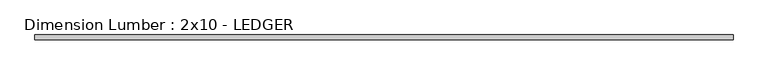
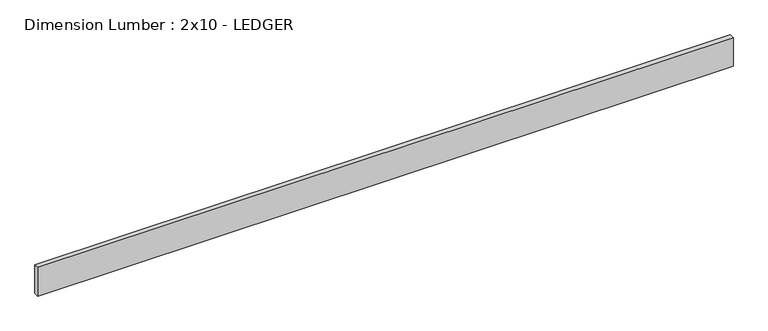
"""IFC4 building model written with IfcOpenShell, lengths in millimetres: beam geometry, Dimension Lumber : 2x10 - LEDGER."""

from ifc_helpers import new_model, si_unit, frame, origin, place, context, project, spatial, polyline, outline, extrude, source, transform, mapped, element, save


def dimension_lumber_2x10_ledger_24f69769(model_context):
    return source(origin(), model_context, "Body", "SweptSolid", [
        extrude(outline(polyline([(2705.1, 19.05), (2705.1, -19.05), (-2705.1, -19.05), (-2705.1, 19.05), (2705.1, 19.05)])), frame((0.0, 0.0, -117.475), z_axis=(0.0, 0.0, 1.0), x_axis=(1.0, 0.0, 0.0)), (0.0, 0.0, 1.0), 234.95),
    ])


if __name__ == "__main__":
    model = new_model("IFC4")
    model_context = context("Model", 3, world=origin())
    ifc_project = project(units=[si_unit("LENGTHUNIT", "METRE", prefix="MILLI")], contexts=[model_context])
    site = spatial("IfcSite", under=ifc_project)
    building = spatial("IfcBuilding", under=site)
    placement = place(None, origin())
    dimension_lumber_2x10_ledger_shape = dimension_lumber_2x10_ledger_24f69769(model_context)
    element("IfcBeam", 1, ObjectType="Dimension Lumber : 2x10 - LEDGER", at=placement, inside=building, context=model_context, shape_type="MappedRepresentation", body=[
        mapped(dimension_lumber_2x10_ledger_shape, transform((0.0, 0.0, 0.0), x_axis=(1.0, 0.0, 0.0), y_axis=(0.0, 1.0, 0.0), z_axis=(0.0, 0.0, 1.0))),
    ])
    save(model, "model.ifc")

# Revit data of these elements
# Type "Dimension Lumber : 2x10 - LEDGER"
#   Assembly Code = "B10"
#   A = 0.0963889 SF
#   Length [instance default] = 5' - 0"
#   b = 0' - 1 1/2"
#   d = 0' - 9 1/4"
#   Structural Material = TREATED 2X10 RIM JOIST
# Element 1 (IfcBeam, "Dimension Lumber : 2x10 - LEDGER")
#   Materials on its faces: "TREATED 2X10 RIM JOIST"
# Materials
#   "TREATED 2X10 RIM JOIST": class "Wood", colour RGB 234 198 147, transparency 0, Description = "Pinus Echinata", Cost = 0
